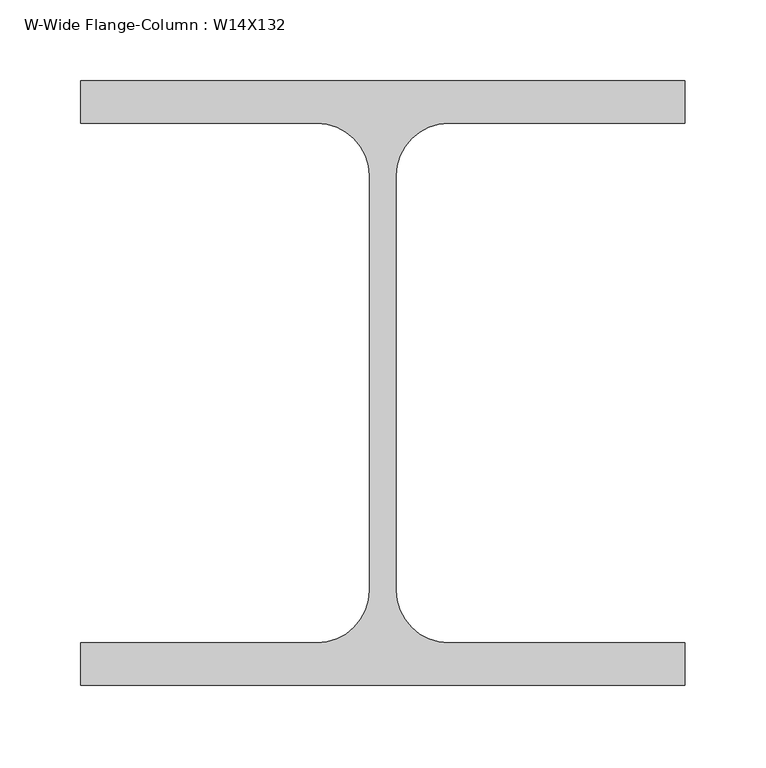
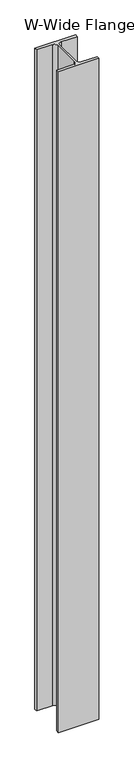
"""IFC4 building model written with IfcOpenShell, lengths in millimetres: column geometry, W-Wide Flange-Column : W14X132."""

from ifc_helpers import new_model, si_unit, point, frame, frame_2d, origin, place, context, project, spatial, polyline, circle_curve, trimmed, segment, composite_curve, outline, extrude, source, transform, mapped, element, save


def w_wide_flange_column_w14x132_b8660559(model_context):
    return source(origin(), model_context, "Body", "SweptSolid", [
        extrude(outline(composite_curve([segment(polyline([(186.69, -186.69), (-186.69, -186.69), (-186.69, -160.528), (-40.767, -160.528)]), True, "CONTINUOUS"), segment(trimmed(circle_curve(frame_2d((-40.767, -127.9525)), 32.5755), [point((-40.767, -160.528))], [point((-8.1915, -127.9525))], True, "CARTESIAN"), True, "CONTINUOUS"), segment(polyline([(-8.1915, -127.9525), (-8.1915, 127.9525)]), True, "CONTINUOUS"), segment(trimmed(circle_curve(frame_2d((-40.767, 127.9525)), 32.5755), [point((-8.1915, 127.9525))], [point((-40.767, 160.528))], True, "CARTESIAN"), True, "CONTINUOUS"), segment(polyline([(-40.767, 160.528), (-186.69, 160.528), (-186.69, 186.69), (186.69, 186.69), (186.69, 160.528), (40.767, 160.528)]), True, "CONTINUOUS"), segment(trimmed(circle_curve(frame_2d((40.767, 127.9525)), 32.5755), [point((40.767, 160.528))], [point((8.1915, 127.9525))], True, "CARTESIAN"), True, "CONTINUOUS"), segment(polyline([(8.1915, 127.9525), (8.1915, -127.9525)]), True, "CONTINUOUS"), segment(trimmed(circle_curve(frame_2d((40.767, -127.9525)), 32.5755), [point((8.1915, -127.9525))], [point((40.767, -160.528))], True, "CARTESIAN"), True, "CONTINUOUS"), segment(polyline([(40.767, -160.528), (186.69, -160.528), (186.69, -186.69)]), True, "CONTINUOUS")], self_intersect=False)), frame((0.0, 0.0, -457.2), z_axis=(0.0, 0.0, 1.0), x_axis=(1.0, 0.0, 0.0)), (0.0, 0.0, 1.0), 6426.2),
    ])


if __name__ == "__main__":
    model = new_model("IFC4")
    model_context = context("Model", 3, world=origin())
    ifc_project = project(units=[si_unit("LENGTHUNIT", "METRE", prefix="MILLI")], contexts=[model_context])
    site = spatial("IfcSite", under=ifc_project)
    building = spatial("IfcBuilding", under=site)
    placement = place(None, origin())
    w_wide_flange_column_w14x132_shape = w_wide_flange_column_w14x132_b8660559(model_context)
    element("IfcColumn", 1, ObjectType="W-Wide Flange-Column : W14X132", at=placement, inside=building, context=model_context, shape_type="MappedRepresentation", body=[
        mapped(w_wide_flange_column_w14x132_shape, transform((0.0, 0.0, 0.0), x_axis=(1.0, 0.0, 0.0), y_axis=(0.0, 1.0, 0.0), z_axis=(0.0, 0.0, 1.0))),
    ])
    save(model, "model.ifc")

# Revit data of these elements
# Type "W-Wide Flange-Column : W14X132"
#   Assembly Code = "B10"
#   W = 132
#   bf = 1' - 2.7"
#   d = 1' - 2.7"
#   k = 0' - 2 5/16"
#   kr = 0' - 1.2825"
#   tf = 0' - 1.03"
#   tw = 0' - 0.645"
#   A = 0.269444 SF
#   Column Material [instance default] = Metal - Steel - ASTM A992
# Element 1 (IfcColumn, "W-Wide Flange-Column : W14X132")
#   Materials on its faces: "Metal - Steel - ASTM A992"
# Materials
#   "Metal - Steel - ASTM A992": class "Metal", colour RGB 128 0 0, transparency 0
